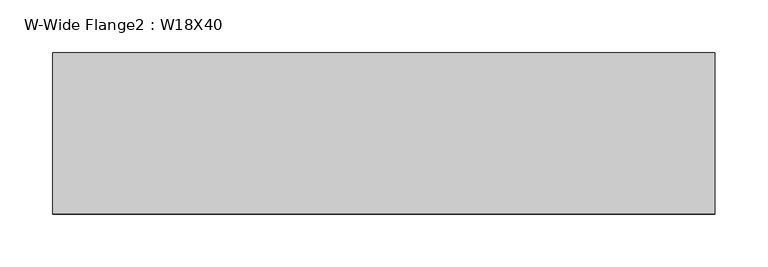
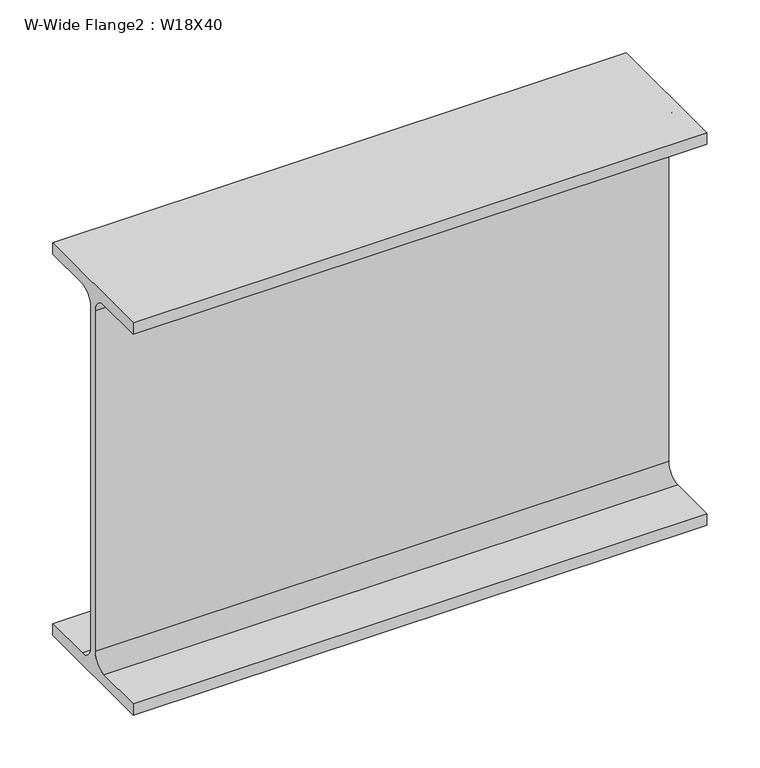
"""IFC4 building model written with IfcOpenShell, lengths in millimetres: beam geometry, W-Wide Flange2 : W18X40."""

import ifcopenshell
import ifcopenshell.guid

model = None  # the IFC model being written
_history = None  # IfcOwnerHistory: only IFC2X3 demands one
_inside = {}  # id of a spatial element -> (the spatial element, [elements in it])
_under = {}  # id of a project, library or spatial element -> (it, [spatial elements below it])
_declared = {}  # id of a project -> (the project, [libraries it declares])
_typed = {}  # id of a type object -> (the type object, [elements of that type])
_made_of = {}  # id of a material, layer set ... -> (it, [elements and type objects made of it])


def new_model(schema):
    """Start an empty IFC model of exactly this schema.

    Asked for "IFC4X3", IfcOpenShell would pick the latest addendum, in which some entities
    have other attributes; the version numbers below select the first issue.
    IFC2X3 requires an IfcOwnerHistory on every rooted entity: one is made here for all.
    """
    global model, _history
    if schema == "IFC4X3":
        model = ifcopenshell.file(schema_version=(4, 3, 0, 0))
    else:
        model = ifcopenshell.file(schema=schema)
    _inside.clear()
    _under.clear()
    _declared.clear()
    _typed.clear()
    _made_of.clear()
    _history = None
    if model.schema == "IFC2X3":
        org = make("IfcOrganization", Name="unknown")
        user = make(
            "IfcPersonAndOrganization",
            ThePerson=make("IfcPerson", FamilyName="unknown"),
            TheOrganization=org,
        )
        app = make(
            "IfcApplication",
            ApplicationDeveloper=org,
            Version="unknown",
            ApplicationFullName="unknown",
            ApplicationIdentifier="unknown",
        )
        _history = make(
            "IfcOwnerHistory",
            OwningUser=user,
            OwningApplication=app,
            ChangeAction="ADDED",
            CreationDate=0,
        )
    return model


def make(cls, **values):
    """One entity of the class cls with the attributes given. An attribute that is None is left unset."""
    return model.create_entity(
        cls, **{name: value for name, value in values.items() if value is not None}
    )


def rooted(cls, **values):
    """An entity with a GlobalId (a new one), such as an element, a storey or a relation."""
    return make(cls, GlobalId=ifcopenshell.guid.new(), OwnerHistory=_history, **values)


def si_unit(unit_type, name, prefix=None):
    """IfcSIUnit, for example si_unit("LENGTHUNIT", "METRE", prefix="MILLI")."""
    return make("IfcSIUnit", UnitType=unit_type, Prefix=prefix, Name=name)


def assignment(units):
    """IfcUnitAssignment: the units of a project."""
    return None if units is None else make("IfcUnitAssignment", Units=units)


def point(xyz):
    """IfcCartesianPoint."""
    return None if xyz is None else make("IfcCartesianPoint", Coordinates=xyz)


def direction(xyz):
    """IfcDirection."""
    return None if xyz is None else make("IfcDirection", DirectionRatios=xyz)


def frame(location, z_axis=None, x_axis=None):
    """IfcAxis2Placement3D, a coordinate frame: its origin and axes. An axis left out is left unset."""
    return make(
        "IfcAxis2Placement3D",
        Location=point(location),
        Axis=direction(z_axis),
        RefDirection=direction(x_axis),
    )


def frame_2d(location, x_axis=None):
    """IfcAxis2Placement2D, a coordinate frame in the plane: its origin and x axis."""
    return make(
        "IfcAxis2Placement2D", Location=point(location), RefDirection=direction(x_axis)
    )


def origin():
    """The frame at (0, 0, 0) with its axes left unset."""
    return frame((0.0, 0.0, 0.0))


def place(relative_to, where):
    """IfcLocalPlacement: puts the frame where relative to a parent placement (None: the world)."""
    return make(
        "IfcLocalPlacement", PlacementRelTo=relative_to, RelativePlacement=where
    )


def context(
    kind, dimensions, precision=None, world=None, true_north=None, identifier=None
):
    """IfcGeometricRepresentationContext, for example the 3D "Model" context."""
    return make(
        "IfcGeometricRepresentationContext",
        ContextIdentifier=identifier,
        ContextType=kind,
        CoordinateSpaceDimension=dimensions,
        Precision=precision,
        WorldCoordinateSystem=world,
        TrueNorth=true_north,
    )


def project(units=None, contexts=None):
    """IfcProject with its units and contexts."""
    return rooted(
        "IfcProject",
        Name="project",
        RepresentationContexts=contexts,
        UnitsInContext=assignment(units),
    )


def spatial(cls, under=None, at=None, **own):
    """A site, building, storey or space (cls), placed at a placement, below another one or the project."""
    s = rooted(cls, ObjectPlacement=at, **own)
    if under is not None:
        _under.setdefault(under.id(), (under, []))[1].append(s)
    return s


def polyline(points):
    """IfcPolyline through the points."""
    return make("IfcPolyline", Points=[point(p) for p in points])


def circle_curve(where, radius):
    """IfcCircle in the frame where."""
    return make("IfcCircle", Position=where, Radius=radius)


def trimmed(basis, trim1, trim2, sense, master):
    """IfcTrimmedCurve: the piece of a basis curve between two trims."""
    return make(
        "IfcTrimmedCurve",
        BasisCurve=basis,
        Trim1=trim1,
        Trim2=trim2,
        SenseAgreement=sense,
        MasterRepresentation=master,
    )


def segment(curve, same_sense, transition):
    """IfcCompositeCurveSegment."""
    return make(
        "IfcCompositeCurveSegment",
        Transition=transition,
        SameSense=same_sense,
        ParentCurve=curve,
    )


def composite_curve(segments, self_intersect=None):
    """IfcCompositeCurve: segments joined end to end."""
    return make("IfcCompositeCurve", Segments=segments, SelfIntersect=self_intersect)


def outline(outer, holes=None, kind="AREA"):
    """IfcArbitraryClosedProfileDef: a profile drawn as a closed curve; with holes, ...WithVoids."""
    if holes is None:
        return make("IfcArbitraryClosedProfileDef", ProfileType=kind, OuterCurve=outer)
    return make(
        "IfcArbitraryProfileDefWithVoids",
        ProfileType=kind,
        OuterCurve=outer,
        InnerCurves=holes,
    )


def extrude(swept, where, along, depth):
    """IfcExtrudedAreaSolid: the profile swept, set in the frame where, extruded along a direction by depth."""
    return make(
        "IfcExtrudedAreaSolid",
        SweptArea=swept,
        Position=where,
        ExtrudedDirection=direction(along),
        Depth=depth,
    )


def shape(context_of_items, identifier, shape_type, items):
    """IfcShapeRepresentation: the items that make up one representation, for example the "Body"."""
    return make(
        "IfcShapeRepresentation",
        ContextOfItems=context_of_items,
        RepresentationIdentifier=identifier,
        RepresentationType=shape_type,
        Items=items,
    )


def source(mapping_origin, context_of_items, identifier, shape_type, items):
    """IfcRepresentationMap: a shape defined once, which mapped items show again and again."""
    return make(
        "IfcRepresentationMap",
        MappingOrigin=mapping_origin,
        MappedRepresentation=shape(context_of_items, identifier, shape_type, items),
    )


def transform(
    local_origin,
    x_axis=None,
    y_axis=None,
    z_axis=None,
    scale=None,
    scale2=None,
    scale3=None,
    uniform=True,
):
    """IfcCartesianTransformationOperator3D, or its non-uniform kind. x_axis, y_axis, z_axis: its Axis1, 2, 3."""
    if uniform:
        return make(
            "IfcCartesianTransformationOperator3D",
            Axis1=direction(x_axis),
            Axis2=direction(y_axis),
            LocalOrigin=point(local_origin),
            Scale=scale,
            Axis3=direction(z_axis),
        )
    return make(
        "IfcCartesianTransformationOperator3DnonUniform",
        Axis1=direction(x_axis),
        Axis2=direction(y_axis),
        LocalOrigin=point(local_origin),
        Scale=scale,
        Axis3=direction(z_axis),
        Scale2=scale2,
        Scale3=scale3,
    )


def mapped(mapping_source, mapping_target):
    """IfcMappedItem: shows the shape of a source again, moved by a transform."""
    return make(
        "IfcMappedItem", MappingSource=mapping_source, MappingTarget=mapping_target
    )


def made_of(thing, what):
    """Note that an element or type object is made of a material, layer set ...; save() writes the relation."""
    if what is not None:
        _made_of.setdefault(what.id(), (what, []))[1].append(thing)
    return thing


def element(
    cls,
    number,
    at=None,
    inside=None,
    cuts=None,
    type_object=None,
    material=None,
    context=None,
    identifier="Body",
    shape_type=None,
    held_by="IfcProductDefinitionShape",
    body=None,
    shapes=None,
    **own,
):
    """One element of the class cls, such as IfcWall. Its Tag is "e" and its number.

    at: its placement. inside: the storey or other place that contains it. cuts: it is an
    opening in that element (IfcRelVoidsElement). A single representation is given by context,
    identifier, shape_type and body (its items); several are given by shapes. held_by: the class
    of the entity that holds the representations. save() writes the other relations.
    """
    e = rooted(cls, Tag="e%d" % number, ObjectPlacement=at, **own)
    if body is not None:
        shapes = [shape(context, identifier, shape_type, body)]
    if shapes is not None:
        e.Representation = make(held_by, Representations=shapes)
    if inside is not None:
        _inside.setdefault(inside.id(), (inside, []))[1].append(e)
    if cuts is not None:
        rooted(
            "IfcRelVoidsElement", RelatingBuildingElement=cuts, RelatedOpeningElement=e
        )
    if type_object is not None:
        _typed.setdefault(type_object.id(), (type_object, []))[1].append(e)
    return made_of(e, material)


def aggregate(whole, parts):
    """IfcRelAggregates: a whole, such as a stair, and the parts it consists of."""
    return rooted("IfcRelAggregates", RelatingObject=whole, RelatedObjects=parts)


def save(model, path):
    """Write the relations noted so far, then the file.

    IfcRelAggregates (storeys below a building ...), IfcRelContainedInSpatialStructure (elements
    in a storey), IfcRelDefinesByType, IfcRelAssociatesMaterial and IfcRelDeclares: one each for
    every whole, place, type object, material and project.
    """
    for whole, parts in _under.values():
        aggregate(whole, parts)
    for where, things in _inside.values():
        rooted(
            "IfcRelContainedInSpatialStructure",
            RelatedElements=things,
            RelatingStructure=where,
        )
    for kind, things in _typed.values():
        rooted("IfcRelDefinesByType", RelatedObjects=things, RelatingType=kind)
    for what, things in _made_of.values():
        rooted("IfcRelAssociatesMaterial", RelatedObjects=things, RelatingMaterial=what)
    for by, libraries in _declared.values():
        rooted("IfcRelDeclares", RelatingContext=by, RelatedDefinitions=libraries)
    model.write(path)


def w_wide_flange2_w18x40_d42051aa(model_context):
    return source(origin(), model_context, "Body", "SweptSolid", [
        extrude(outline(composite_curve([segment(polyline([(76.454, -213.995), (76.454, -227.33), (-76.454, -227.33), (-76.454, -213.995), (-20.828, -213.995)]), True, "CONTINUOUS"), segment(trimmed(circle_curve(frame_2d((-20.828, -197.1675)), 16.8275), [point((-20.828, -213.995))], [point((-4.0005, -197.1675))], True, "CARTESIAN"), True, "CONTINUOUS"), segment(polyline([(-4.0005, -197.1675), (-4.0005, 197.1675)]), True, "CONTINUOUS"), segment(trimmed(circle_curve(frame_2d((-20.828, 197.1675)), 16.8275), [point((-4.0005, 197.1675))], [point((-20.828, 213.995))], True, "CARTESIAN"), True, "CONTINUOUS"), segment(polyline([(-20.828, 213.995), (-76.454, 213.995), (-76.454, 227.33), (76.454, 227.33), (76.454, 213.995), (20.828, 213.995)]), True, "CONTINUOUS"), segment(trimmed(circle_curve(frame_2d((20.828, 197.1675)), 16.8275), [point((20.828, 213.995))], [point((4.0005, 197.1675))], True, "CARTESIAN"), True, "CONTINUOUS"), segment(polyline([(4.0005, 197.1675), (4.0005, -197.1675)]), True, "CONTINUOUS"), segment(trimmed(circle_curve(frame_2d((20.828, -197.1675)), 16.8275), [point((4.0005, -197.1675))], [point((20.828, -213.995))], True, "CARTESIAN"), True, "CONTINUOUS"), segment(polyline([(20.828, -213.995), (76.454, -213.995)]), True, "CONTINUOUS")], self_intersect=False)), frame((-345.28125, 0.0, 0.0), z_axis=(1.0, 0.0, 0.0), x_axis=(0.0, 1.0, 0.0)), (0.0, 0.0, 1.0), 628.253125),
    ])


if __name__ == "__main__":
    model = new_model("IFC4")
    model_context = context("Model", 3, world=origin())
    ifc_project = project(units=[si_unit("LENGTHUNIT", "METRE", prefix="MILLI")], contexts=[model_context])
    site = spatial("IfcSite", under=ifc_project)
    building = spatial("IfcBuilding", under=site)
    placement = place(None, origin())
    w_wide_flange2_w18x40_shape = w_wide_flange2_w18x40_d42051aa(model_context)
    element("IfcBeam", 1, ObjectType="W-Wide Flange2 : W18X40", at=placement, inside=building, context=model_context, shape_type="MappedRepresentation", body=[
        mapped(w_wide_flange2_w18x40_shape, transform((0.0, 0.0, 0.0), x_axis=(1.0, 0.0, 0.0), y_axis=(0.0, 1.0, 0.0), z_axis=(0.0, 0.0, 1.0))),
    ])
    save(model, "model.ifc")

# Revit data of these elements
# Type "W-Wide Flange2 : W18X40"
#   Assembly Code = "B10"
#   W = 40
#   Length [instance default] = 5' - 0"
#   bf = 0' - 6.02"
#   d = 1' - 5.9"
#   k = 0' - 1 3/16"
#   k2 = 0' - 0.6625"
#   tf = 0' - 0.525"
#   tw = 0' - 0.315"
#   A = 0.0819444 SF
#   Structural Material [instance default] = Steel ASTM A992
# Element 1 (IfcBeam, "W-Wide Flange2 : W18X40")
#   Materials on its faces: "Steel ASTM A992"
# Materials
#   "Steel ASTM A992": class "Metal", colour RGB 199 199 199, transparency 0, Description = "Structural steel 50ksi", Cost = 0
